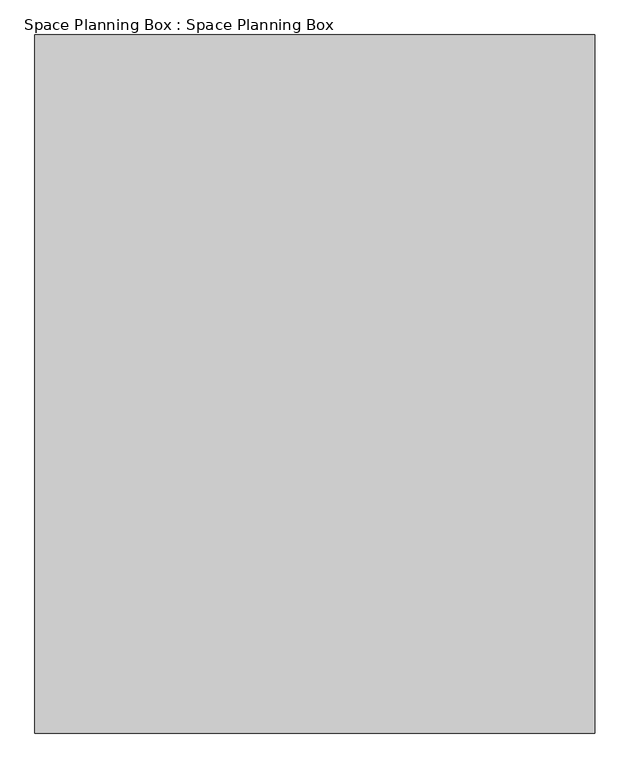
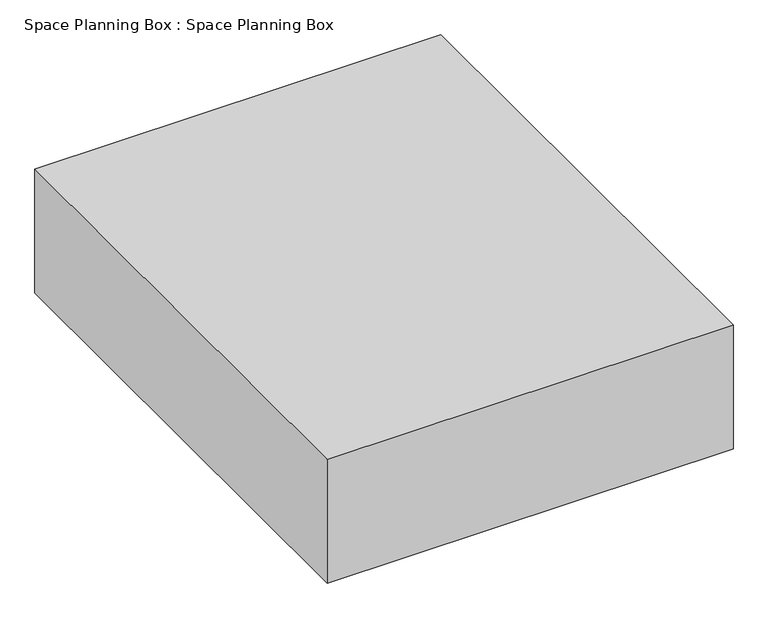
"""IFC4 building model written with IfcOpenShell, lengths in millimetres: proxy geometry, Space Planning Box : Space Planning Box."""

from ifc_helpers import new_model, si_unit, origin, origin_with_axes, place, context, project, spatial, polyline, outline, extrude, source, transform, mapped, element, save


def space_planning_box_space_planning_box_d82b1902(model_context):
    return source(origin(), model_context, "Body", "SweptSolid", [
        extrude(outline(polyline([(9300.0, 11600.0), (9300.0, -11600.0), (-9300.0, -11600.0), (-9300.0, 11600.0), (9300.0, 11600.0)])), origin_with_axes(), (0.0, 0.0, 1.0), 6000.0),
    ])


if __name__ == "__main__":
    model = new_model("IFC4")
    model_context = context("Model", 3, world=origin())
    ifc_project = project(units=[si_unit("LENGTHUNIT", "METRE", prefix="MILLI")], contexts=[model_context])
    site = spatial("IfcSite", under=ifc_project)
    building = spatial("IfcBuilding", under=site)
    placement = place(None, origin())
    space_planning_box_space_planning_box_shape = space_planning_box_space_planning_box_d82b1902(model_context)
    element("IfcBuildingElementProxy", 1, Name="Space Planning Box : Space Planning Box", ObjectType="Space Planning Box : Space Planning Box", at=placement, inside=building, context=model_context, shape_type="MappedRepresentation", body=[
        mapped(space_planning_box_space_planning_box_shape, transform((0.0, 0.0, 0.0), x_axis=(1.0, 0.0, 0.0), y_axis=(0.0, 1.0, 0.0), z_axis=(0.0, 0.0, 1.0))),
    ])
    save(model, "model.ifc")

# Revit data of these elements
# Type "Space Planning Box : Space Planning Box"
#   Type Comments = "..."
#   Room Name [instance default] = "?"
#   Assembly Code = "..."
#   Width [instance default] = 1524 mm
#   Program Area [instance default] = 0 m²
#   Length [instance default] = 1524 mm
#   Height [instance default] = 1524 mm
#   Area [instance default] = 2.32258 m²
#   Fill Color [instance default] = Cyan
#   Default Elevation = 0
# Element 1 (IfcBuildingElementProxy, "Space Planning Box : Space Planning Box")
#   Room Name = "Electronic Room"
#   Width = 18600 mm
#   Program Area = 431.52 m²
#   Length = 23200 mm
#   Height = 6000 mm
#   Area = 431.52 m²
#   Fill Color = Lime
#   Materials on its faces: "Lime"
# Materials
#   "Cyan": class "Generic", colour RGB 0 255 255, transparency 0.2, Cost = 0
#   "Lime": class "Generic", colour RGB 0 255 0, transparency 0.2, Cost = 0
